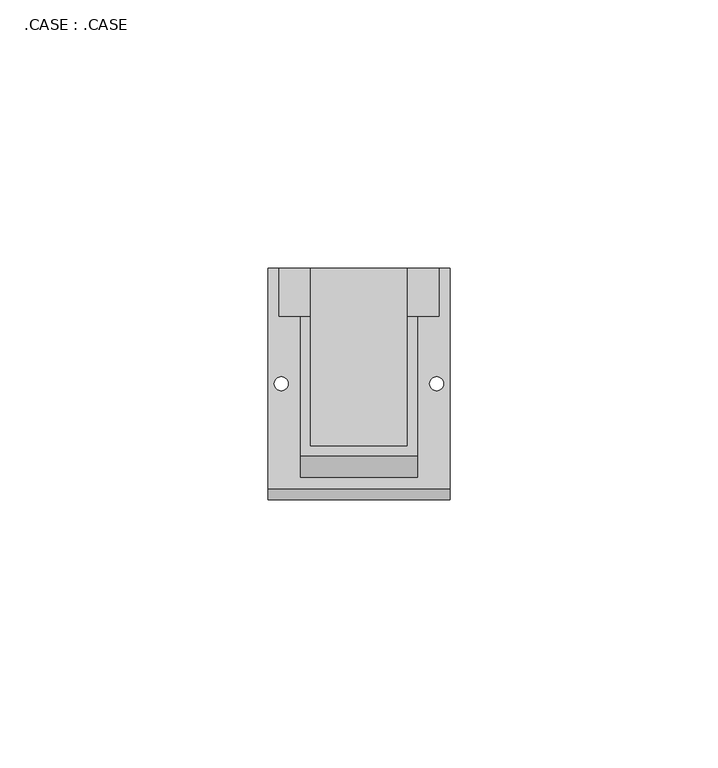
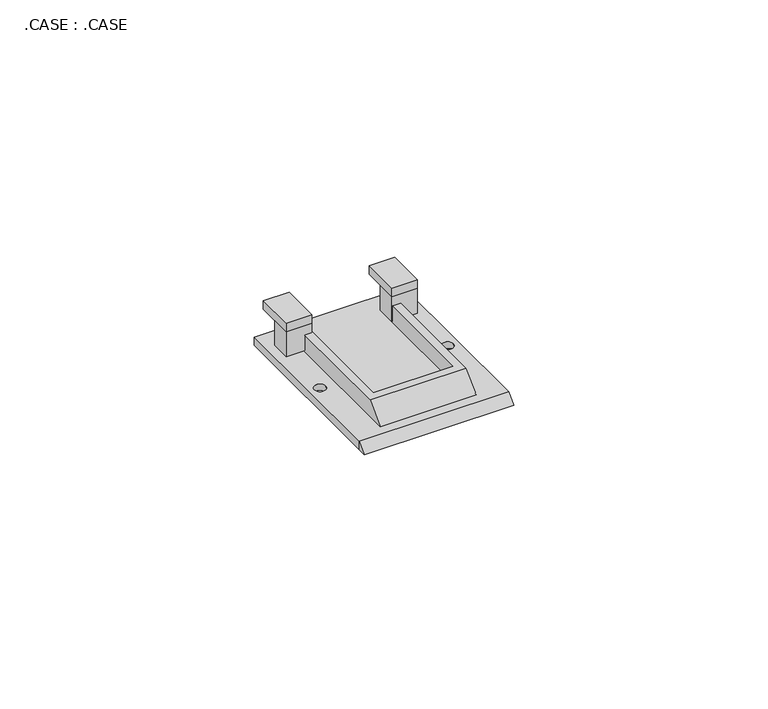
"""IFC4 building model written with IfcOpenShell, lengths in millimetres: proxy geometry, .CASE : .CASE."""

from ifc_helpers import new_model, si_unit, frame, origin, place, context, project, spatial, polyline, circle_curve, outline, extrude, source, transform, mapped, element, save
from ifc_brep_helpers import plane_surface, revolved_surface, advanced_brep


def case_case_62cccb9e(model_context):
    return source(origin(), model_context, "Body", "SolidModel", [
        extrude(outline(polyline([(1442.9350176, 13234.6739696), (1442.9350176, 13225.7186096), (1437.1350176, 13225.7186096), (1437.1350176, 13234.6739696), (1442.9350176, 13234.6739696)])), frame((0.0, 0.0, 8.0), z_axis=(0.0, 0.0, 1.0), x_axis=(1.0, 0.0, 0.0)), (0.0, 0.0, 1.0), 2.0),
        extrude(outline(polyline([(1461.1150176, 13234.6739696), (1466.9150176, 13234.6739696), (1466.9150176, 13225.7186096), (1461.1150176, 13225.7186096), (1461.1150176, 13234.6739696)])), frame((0.0, 0.0, 8.0), z_axis=(0.0, 0.0, 1.0), x_axis=(1.0, 0.0, 0.0)), (0.0, 0.0, 1.0), 2.0),
        extrude(outline(polyline([(1442.9350176, 13230.2186096), (1442.9350176, 13225.7186096), (1437.1350176, 13225.7186096), (1437.1350176, 13230.2186096), (1442.9350176, 13230.2186096)])), frame((0.0, 0.0, 2.0), z_axis=(0.0, 0.0, 1.0), x_axis=(1.0, 0.0, 0.0)), (0.0, 0.0, 1.0), 6.0),
        extrude(outline(polyline([(13191.4256546, 0.0), (13193.4256546, 2.0), (13193.4256546, 0.0), (13191.4256546, 0.0)])), frame((1435.0250176, 0.0, 0.0), z_axis=(1.0, 0.0, 0.0), x_axis=(0.0, 1.0, 0.0)), (0.0, 0.0, 1.0), 34.0),
        extrude(outline(polyline([(1461.1150176, 13230.2186096), (1466.9150176, 13230.2186096), (1466.9150176, 13225.7186096), (1461.1150176, 13225.7186096), (1461.1150176, 13230.2186096)])), frame((0.0, 0.0, 2.0), z_axis=(0.0, 0.0, 1.0), x_axis=(1.0, 0.0, 0.0)), (0.0, 0.0, 1.0), 6.0),
        advanced_brep(
        [(1435.0250176, 13193.4256546, 2.0), (1469.0250176, 13193.4256546, 2.0), (1469.0250176, 13234.6739696, 2.0), (1435.0250176, 13234.6739696, 2.0), (1441.1350176, 13195.6739696, 2.0), (1441.1350176, 13225.7186096, 2.0), (1442.9350176, 13225.7186096, 2.0), (1442.9350176, 13201.4739696, 2.0), (1461.1150176, 13201.4739696, 2.0), (1461.1150176, 13225.7186096, 2.0), (1462.9150176, 13225.7186096, 2.0), (1462.9150176, 13195.6739696, 2.0), (1467.8250176, 13213.1041412, 2.0), (1465.2250176, 13213.1041412, 2.0), (1438.8250176, 13213.1041412, 2.0), (1436.2250176, 13213.1041412, 2.0), (1435.0250176, 13193.4256546, 0.0), (1435.0250176, 13234.6739696, 0.0), (1469.0250176, 13234.6739696, 0.0), (1469.0250176, 13193.4256546, 0.0), (1464.5250176, 13213.1041412, 0.0), (1468.5250176, 13213.1041412, 0.0), (1435.5250176, 13213.1041412, 0.0), (1439.5250176, 13213.1041412, 0.0), (1441.1350176, 13225.7186096, 6.0), (1441.1350176, 13199.6739696, 6.0), (1462.9150176, 13199.6739696, 6.0), (1462.9150176, 13225.7186096, 6.0), (1461.1150176, 13225.7186096, 6.0), (1461.1150176, 13201.4739696, 6.0), (1442.9350176, 13201.4739696, 6.0), (1442.9350176, 13225.7186096, 6.0)],
        [
            (0, 1),
            (1, 2),
            (2, 3),
            (3, 0),
            (4, 5),
            (5, 6),
            (6, 7),
            (7, 8),
            (8, 9),
            (9, 10),
            (10, 11),
            (11, 4),
            (12, 13, circle_curve(frame((1466.5250176, 13213.1041412, 2.0), z_axis=(0.0, 0.0, -1.0), x_axis=(-1.0, 0.0, 0.0)), 1.3)),
            (13, 12, circle_curve(frame((1466.5250176, 13213.1041412, 2.0), z_axis=(0.0, 0.0, -1.0), x_axis=(1.0, 0.0, 0.0)), 1.3)),
            (14, 15, circle_curve(frame((1437.5250176, 13213.1041412, 2.0), z_axis=(0.0, 0.0, -1.0), x_axis=(-1.0, 0.0, 0.0)), 1.3)),
            (15, 14, circle_curve(frame((1437.5250176, 13213.1041412, 2.0), z_axis=(0.0, 0.0, -1.0), x_axis=(1.0, 0.0, 0.0)), 1.3)),
            (16, 17),
            (17, 18),
            (18, 19),
            (19, 16),
            (20, 21, circle_curve(frame((1466.5250176, 13213.1041412, 0.0), z_axis=(0.0, 0.0, 1.0), x_axis=(-1.0, 0.0, 0.0)), 2.0)),
            (21, 20, circle_curve(frame((1466.5250176, 13213.1041412, 0.0), z_axis=(0.0, 0.0, 1.0), x_axis=(1.0, 0.0, 0.0)), 2.0)),
            (22, 23, circle_curve(frame((1437.5250176, 13213.1041412, 0.0), z_axis=(0.0, 0.0, 1.0), x_axis=(-1.0, 0.0, 0.0)), 2.0)),
            (23, 22, circle_curve(frame((1437.5250176, 13213.1041412, 0.0), z_axis=(0.0, 0.0, 1.0), x_axis=(1.0, 0.0, 0.0)), 2.0)),
            (0, 16),
            (19, 1),
            (18, 2),
            (17, 3),
            (24, 25),
            (25, 26),
            (26, 27),
            (27, 28),
            (28, 29),
            (29, 30),
            (30, 31),
            (31, 24),
            (24, 5),
            (4, 25),
            (26, 11),
            (10, 27),
            (9, 28),
            (8, 29),
            (7, 30),
            (6, 31),
            (20, 13),
            (12, 21),
            (22, 15),
            (14, 23),
        ],
        [
            plane_surface(frame((1467.7850176, 13193.4256546, 2.0), z_axis=(0.0, 0.0, 1.0), x_axis=(1.0, 0.0, 0.0))),
            plane_surface(frame((1467.7850176, 13193.4256546, 0.0), z_axis=(0.0, 0.0, -1.0), x_axis=(-1.0, 0.0, 0.0))),
            plane_surface(frame((1435.0250176, 13193.4256546, 2.0), z_axis=(0.0, -1.0, 0.0), x_axis=(0.0, 0.0, -1.0))),
            plane_surface(frame((1469.0250176, 13193.4256546, 2.0), z_axis=(1.0, 0.0, 0.0), x_axis=(0.0, 0.0, -1.0))),
            plane_surface(frame((1469.0250176, 13234.6739696, 2.0), z_axis=(0.0, 1.0, 0.0), x_axis=(0.0, 0.0, -1.0))),
            plane_surface(frame((1435.0250176, 13234.6739696, 2.0), z_axis=(-1.0, 0.0, 0.0), x_axis=(0.0, 0.0, -1.0))),
            plane_surface(frame((1441.1350176, 13234.6739696, 6.0), z_axis=(0.0, 0.0, 1.0), x_axis=(0.0, -1.0, 0.0))),
            plane_surface(frame((1441.1350176, 13225.7186096, 6.0), z_axis=(-1.0, 0.0, 0.0), x_axis=(0.0, 0.0, -1.0))),
            plane_surface(frame((1462.9150176, 13199.6739696, 6.0), z_axis=(1.0, 0.0, 0.0), x_axis=(0.0, 0.0, -1.0))),
            plane_surface(frame((1462.9150176, 13225.7186096, 6.0), z_axis=(0.0, 1.0, 0.0), x_axis=(0.0, 0.0, -1.0))),
            plane_surface(frame((1461.1150176, 13225.7186096, 6.0), z_axis=(-1.0, 0.0, 0.0), x_axis=(0.0, 0.0, -1.0))),
            plane_surface(frame((1461.1150176, 13201.4739696, 6.0), z_axis=(0.0, 1.0, 0.0), x_axis=(0.0, 0.0, -1.0))),
            plane_surface(frame((1442.9350176, 13201.4739696, 6.0), z_axis=(1.0, 0.0, 0.0), x_axis=(0.0, 0.0, -1.0))),
            plane_surface(frame((1442.9350176, 13225.7186096, 6.0), z_axis=(0.0, 1.0, 0.0), x_axis=(0.0, 0.0, -1.0))),
            plane_surface(frame((1441.1350176, 13195.6739696, 2.0), z_axis=(0.0, -0.7071067811865885, 0.7071067811865066), x_axis=(1.0, 0.0, 0.0))),
            revolved_surface(polyline([(1464.5250176, 13213.1041412, 0.0), (1465.2250176017499, 13213.1041412, 2.0)]), (1466.5250176, 13213.1041412, 5.7142857), (0.0, 0.0, -1.0)),
            revolved_surface(polyline([(1435.5250176, 13213.1041412, 0.0), (1436.2250176017499, 13213.1041412, 2.0)]), (1437.5250176, 13213.1041412, 5.7142857), (0.0, 0.0, -1.0)),
        ],
        [
            (0, [[1, 2, 3, 4], [5, 6, 7, 8, 9, 10, 11, 12], [13, 14], [15, 16]]),
            (1, [[17, 18, 19, 20], [21, 22], [23, 24]]),
            (2, [[-1, 25, -20, 26]]),
            (3, [[-2, -26, -19, 27]]),
            (4, [[-3, -27, -18, 28]]),
            (5, [[-4, -28, -17, -25]]),
            (6, [[29, 30, 31, 32, 33, 34, 35, 36]]),
            (7, [[-29, 37, -5, 38]]),
            (8, [[-31, 39, -11, 40]]),
            (9, [[-32, -40, -10, 41]]),
            (10, [[-33, -41, -9, 42]]),
            (11, [[-34, -42, -8, 43]]),
            (12, [[-35, -43, -7, 44]]),
            (13, [[-36, -44, -6, -37]]),
            (14, [[-38, -12, -39, -30]]),
            (15, [[45, -13, 46, -21]]),
            (15, [[-45, -22, -46, -14]]),
            (16, [[47, -15, 48, -23]]),
            (16, [[-47, -24, -48, -16]]),
        ],
    ),
    ])


if __name__ == "__main__":
    model = new_model("IFC4")
    model_context = context("Model", 3, world=origin())
    ifc_project = project(units=[si_unit("LENGTHUNIT", "METRE", prefix="MILLI")], contexts=[model_context])
    site = spatial("IfcSite", under=ifc_project)
    building = spatial("IfcBuilding", under=site)
    placement = place(None, origin())
    case_case_shape = case_case_62cccb9e(model_context)
    element("IfcBuildingElementProxy", 1, Name=".CASE : .CASE", ObjectType=".CASE : .CASE", at=placement, inside=building, context=model_context, shape_type="MappedRepresentation", body=[
        mapped(case_case_shape, transform((0.0, 0.0, 0.0), x_axis=(1.0, 0.0, 0.0), y_axis=(0.0, 1.0, 0.0), z_axis=(0.0, 0.0, 1.0))),
    ])
    save(model, "model.ifc")

# Revit data of these elements
# Project information
#   Data de emissão do projeto = "Data de emissão"
#   Status do projeto = "Status do projeto"
#   Nome do cliente = "Proprietário"
#   Endereço do projeto = "Insira aqui o endereço"
#   Nome do projeto = "Nome do projeto"
#   Número do projeto = "0001"
# Element 1 (IfcBuildingElementProxy, ".CASE : .CASE")
#   Materials on its faces: "Areia"
# Materials
#   "Areia": class "Genérico", colour RGB 191 183 178, transparency 0, Description = "Areia", Cost = 0
